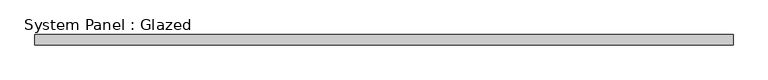
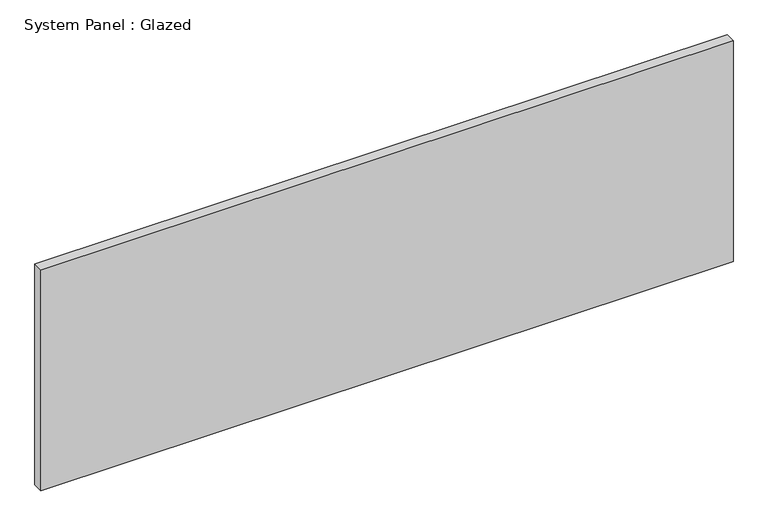
"""IFC4 building model written with IfcOpenShell, lengths in millimetres: plate geometry, System Panel : Glazed."""

from ifc_helpers import new_model, si_unit, origin, origin_with_axes, place, context, project, spatial, polyline, outline, extrude, source, transform, mapped, element, save


def system_panel_glazed_1e4093cb(model_context):
    return source(origin(), model_context, "Body", "SweptSolid", [
        extrude(outline(polyline([(851.3636364, 24.5), (-851.3636364, 24.5), (-851.3636364, 49.5), (851.3636364, 49.5), (851.3636364, 24.5)])), origin_with_axes(), (0.0, 0.0, 1.0), 575.0),
    ])


if __name__ == "__main__":
    model = new_model("IFC4")
    model_context = context("Model", 3, world=origin())
    ifc_project = project(units=[si_unit("LENGTHUNIT", "METRE", prefix="MILLI")], contexts=[model_context])
    site = spatial("IfcSite", under=ifc_project)
    building = spatial("IfcBuilding", under=site)
    placement = place(None, origin())
    system_panel_glazed_shape = system_panel_glazed_1e4093cb(model_context)
    element("IfcPlate", 1, ObjectType="System Panel : Glazed", at=placement, inside=building, context=model_context, shape_type="MappedRepresentation", body=[
        mapped(system_panel_glazed_shape, transform((0.0, 0.0, 0.0), x_axis=(1.0, 0.0, 0.0), y_axis=(0.0, 1.0, 0.0), z_axis=(0.0, 0.0, 1.0))),
    ])
    save(model, "model.ifc")

# Revit data of these elements
# Element 1 (IfcPlate, "System Panel : Glazed")
#   Materials on its faces: "Glass"
# Materials
#   "Glass": class "Glass", colour RGB 218 227 224, transparency 0.85, Description = "Soda Lime Glass", Cost = 0
